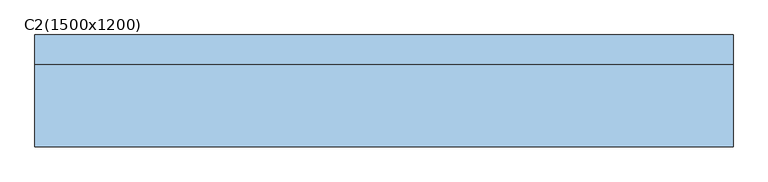
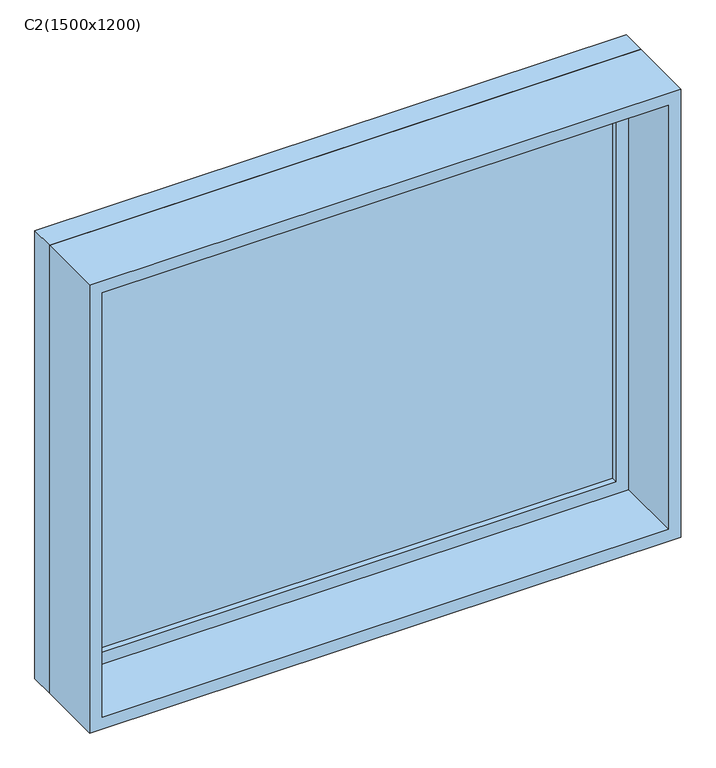
"""IFC4 building model written with IfcOpenShell, lengths in millimetres: window geometry, 固定窗 : C2(1500x1200)."""

import ifcopenshell
import ifcopenshell.guid

model = None  # the IFC model being written
_history = None  # IfcOwnerHistory: only IFC2X3 demands one
_inside = {}  # id of a spatial element -> (the spatial element, [elements in it])
_under = {}  # id of a project, library or spatial element -> (it, [spatial elements below it])
_declared = {}  # id of a project -> (the project, [libraries it declares])
_typed = {}  # id of a type object -> (the type object, [elements of that type])
_made_of = {}  # id of a material, layer set ... -> (it, [elements and type objects made of it])


def new_model(schema):
    """Start an empty IFC model of exactly this schema.

    Asked for "IFC4X3", IfcOpenShell would pick the latest addendum, in which some entities
    have other attributes; the version numbers below select the first issue.
    IFC2X3 requires an IfcOwnerHistory on every rooted entity: one is made here for all.
    """
    global model, _history
    if schema == "IFC4X3":
        model = ifcopenshell.file(schema_version=(4, 3, 0, 0))
    else:
        model = ifcopenshell.file(schema=schema)
    _inside.clear()
    _under.clear()
    _declared.clear()
    _typed.clear()
    _made_of.clear()
    _history = None
    if model.schema == "IFC2X3":
        org = make("IfcOrganization", Name="unknown")
        user = make(
            "IfcPersonAndOrganization",
            ThePerson=make("IfcPerson", FamilyName="unknown"),
            TheOrganization=org,
        )
        app = make(
            "IfcApplication",
            ApplicationDeveloper=org,
            Version="unknown",
            ApplicationFullName="unknown",
            ApplicationIdentifier="unknown",
        )
        _history = make(
            "IfcOwnerHistory",
            OwningUser=user,
            OwningApplication=app,
            ChangeAction="ADDED",
            CreationDate=0,
        )
    return model


def make(cls, **values):
    """One entity of the class cls with the attributes given. An attribute that is None is left unset."""
    return model.create_entity(
        cls, **{name: value for name, value in values.items() if value is not None}
    )


def rooted(cls, **values):
    """An entity with a GlobalId (a new one), such as an element, a storey or a relation."""
    return make(cls, GlobalId=ifcopenshell.guid.new(), OwnerHistory=_history, **values)


def si_unit(unit_type, name, prefix=None):
    """IfcSIUnit, for example si_unit("LENGTHUNIT", "METRE", prefix="MILLI")."""
    return make("IfcSIUnit", UnitType=unit_type, Prefix=prefix, Name=name)


def assignment(units):
    """IfcUnitAssignment: the units of a project."""
    return None if units is None else make("IfcUnitAssignment", Units=units)


def point(xyz):
    """IfcCartesianPoint."""
    return None if xyz is None else make("IfcCartesianPoint", Coordinates=xyz)


def direction(xyz):
    """IfcDirection."""
    return None if xyz is None else make("IfcDirection", DirectionRatios=xyz)


def frame(location, z_axis=None, x_axis=None):
    """IfcAxis2Placement3D, a coordinate frame: its origin and axes. An axis left out is left unset."""
    return make(
        "IfcAxis2Placement3D",
        Location=point(location),
        Axis=direction(z_axis),
        RefDirection=direction(x_axis),
    )


def origin():
    """The frame at (0, 0, 0) with its axes left unset."""
    return frame((0.0, 0.0, 0.0))


def place(relative_to, where):
    """IfcLocalPlacement: puts the frame where relative to a parent placement (None: the world)."""
    return make(
        "IfcLocalPlacement", PlacementRelTo=relative_to, RelativePlacement=where
    )


def context(
    kind, dimensions, precision=None, world=None, true_north=None, identifier=None
):
    """IfcGeometricRepresentationContext, for example the 3D "Model" context."""
    return make(
        "IfcGeometricRepresentationContext",
        ContextIdentifier=identifier,
        ContextType=kind,
        CoordinateSpaceDimension=dimensions,
        Precision=precision,
        WorldCoordinateSystem=world,
        TrueNorth=true_north,
    )


def project(units=None, contexts=None):
    """IfcProject with its units and contexts."""
    return rooted(
        "IfcProject",
        Name="project",
        RepresentationContexts=contexts,
        UnitsInContext=assignment(units),
    )


def spatial(cls, under=None, at=None, **own):
    """A site, building, storey or space (cls), placed at a placement, below another one or the project."""
    s = rooted(cls, ObjectPlacement=at, **own)
    if under is not None:
        _under.setdefault(under.id(), (under, []))[1].append(s)
    return s


def polyline(points):
    """IfcPolyline through the points."""
    return make("IfcPolyline", Points=[point(p) for p in points])


def outline(outer, holes=None, kind="AREA"):
    """IfcArbitraryClosedProfileDef: a profile drawn as a closed curve; with holes, ...WithVoids."""
    if holes is None:
        return make("IfcArbitraryClosedProfileDef", ProfileType=kind, OuterCurve=outer)
    return make(
        "IfcArbitraryProfileDefWithVoids",
        ProfileType=kind,
        OuterCurve=outer,
        InnerCurves=holes,
    )


def extrude(swept, where, along, depth):
    """IfcExtrudedAreaSolid: the profile swept, set in the frame where, extruded along a direction by depth."""
    return make(
        "IfcExtrudedAreaSolid",
        SweptArea=swept,
        Position=where,
        ExtrudedDirection=direction(along),
        Depth=depth,
    )


def shape(context_of_items, identifier, shape_type, items):
    """IfcShapeRepresentation: the items that make up one representation, for example the "Body"."""
    return make(
        "IfcShapeRepresentation",
        ContextOfItems=context_of_items,
        RepresentationIdentifier=identifier,
        RepresentationType=shape_type,
        Items=items,
    )


def source(mapping_origin, context_of_items, identifier, shape_type, items):
    """IfcRepresentationMap: a shape defined once, which mapped items show again and again."""
    return make(
        "IfcRepresentationMap",
        MappingOrigin=mapping_origin,
        MappedRepresentation=shape(context_of_items, identifier, shape_type, items),
    )


def transform(
    local_origin,
    x_axis=None,
    y_axis=None,
    z_axis=None,
    scale=None,
    scale2=None,
    scale3=None,
    uniform=True,
):
    """IfcCartesianTransformationOperator3D, or its non-uniform kind. x_axis, y_axis, z_axis: its Axis1, 2, 3."""
    if uniform:
        return make(
            "IfcCartesianTransformationOperator3D",
            Axis1=direction(x_axis),
            Axis2=direction(y_axis),
            LocalOrigin=point(local_origin),
            Scale=scale,
            Axis3=direction(z_axis),
        )
    return make(
        "IfcCartesianTransformationOperator3DnonUniform",
        Axis1=direction(x_axis),
        Axis2=direction(y_axis),
        LocalOrigin=point(local_origin),
        Scale=scale,
        Axis3=direction(z_axis),
        Scale2=scale2,
        Scale3=scale3,
    )


def mapped(mapping_source, mapping_target):
    """IfcMappedItem: shows the shape of a source again, moved by a transform."""
    return make(
        "IfcMappedItem", MappingSource=mapping_source, MappingTarget=mapping_target
    )


def made_of(thing, what):
    """Note that an element or type object is made of a material, layer set ...; save() writes the relation."""
    if what is not None:
        _made_of.setdefault(what.id(), (what, []))[1].append(thing)
    return thing


def element(
    cls,
    number,
    at=None,
    inside=None,
    cuts=None,
    type_object=None,
    material=None,
    context=None,
    identifier="Body",
    shape_type=None,
    held_by="IfcProductDefinitionShape",
    body=None,
    shapes=None,
    **own,
):
    """One element of the class cls, such as IfcWall. Its Tag is "e" and its number.

    at: its placement. inside: the storey or other place that contains it. cuts: it is an
    opening in that element (IfcRelVoidsElement). A single representation is given by context,
    identifier, shape_type and body (its items); several are given by shapes. held_by: the class
    of the entity that holds the representations. save() writes the other relations.
    """
    e = rooted(cls, Tag="e%d" % number, ObjectPlacement=at, **own)
    if body is not None:
        shapes = [shape(context, identifier, shape_type, body)]
    if shapes is not None:
        e.Representation = make(held_by, Representations=shapes)
    if inside is not None:
        _inside.setdefault(inside.id(), (inside, []))[1].append(e)
    if cuts is not None:
        rooted(
            "IfcRelVoidsElement", RelatingBuildingElement=cuts, RelatedOpeningElement=e
        )
    if type_object is not None:
        _typed.setdefault(type_object.id(), (type_object, []))[1].append(e)
    return made_of(e, material)


def aggregate(whole, parts):
    """IfcRelAggregates: a whole, such as a stair, and the parts it consists of."""
    return rooted("IfcRelAggregates", RelatingObject=whole, RelatedObjects=parts)


def save(model, path):
    """Write the relations noted so far, then the file.

    IfcRelAggregates (storeys below a building ...), IfcRelContainedInSpatialStructure (elements
    in a storey), IfcRelDefinesByType, IfcRelAssociatesMaterial and IfcRelDeclares: one each for
    every whole, place, type object, material and project.
    """
    for whole, parts in _under.values():
        aggregate(whole, parts)
    for where, things in _inside.values():
        rooted(
            "IfcRelContainedInSpatialStructure",
            RelatedElements=things,
            RelatingStructure=where,
        )
    for kind, things in _typed.values():
        rooted("IfcRelDefinesByType", RelatedObjects=things, RelatingType=kind)
    for what, things in _made_of.values():
        rooted("IfcRelAssociatesMaterial", RelatedObjects=things, RelatingMaterial=what)
    for by, libraries in _declared.values():
        rooted("IfcRelDeclares", RelatingContext=by, RelatedDefinitions=libraries)
    model.write(path)


def c2_1500x1200_cfff0f4c(model_context):
    return source(origin(), model_context, "Body", "SweptSolid", [
        extrude(outline(polyline([(648.4, 71.425), (-724.6, 71.425), (-724.6, 84.125), (648.4, 84.125), (648.4, 71.425)])), frame((0.0, 0.0, 963.5), z_axis=(0.0, 0.0, 1.0), x_axis=(1.0, 0.0, 0.0)), (0.0, 0.0, 1.0), 1073.0),
        extrude(outline(polyline([(2080.95, -769.05), (919.05, -769.05), (919.05, 692.85), (2080.95, 692.85), (2080.95, -769.05)]), holes=[polyline([(2036.5, -724.6), (2036.5, 648.4), (963.5, 648.4), (963.5, -724.6), (2036.5, -724.6)])]), frame((0.0, 55.55, 0.0), z_axis=(0.0, 1.0, 0.0), x_axis=(0.0, 0.0, 1.0)), (0.0, 0.0, 1.0), 44.45),
        extrude(outline(polyline([(2100.0, -788.1), (900.0, -788.1), (900.0, 711.9), (2100.0, 711.9), (2100.0, -788.1)]), holes=[polyline([(2068.25, -756.35), (2068.25, 680.15), (931.75, 680.15), (931.75, -756.35), (2068.25, -756.35)])]), frame((0.0, -120.0, 0.0), z_axis=(0.0, 1.0, 0.0), x_axis=(0.0, 0.0, 1.0)), (0.0, 0.0, 1.0), 175.55),
        extrude(outline(polyline([(2100.0, 711.9), (2100.0, -788.1), (900.0, -788.1), (900.0, 711.9), (2100.0, 711.9)]), holes=[polyline([(2080.95, 692.85), (919.05, 692.85), (919.05, -769.05), (2080.95, -769.05), (2080.95, 692.85)])]), frame((0.0, 55.55, 0.0), z_axis=(0.0, 1.0, 0.0), x_axis=(0.0, 0.0, 1.0)), (0.0, 0.0, 1.0), 64.45),
    ])


if __name__ == "__main__":
    model = new_model("IFC4")
    model_context = context("Model", 3, world=origin())
    ifc_project = project(units=[si_unit("LENGTHUNIT", "METRE", prefix="MILLI")], contexts=[model_context])
    site = spatial("IfcSite", under=ifc_project)
    building = spatial("IfcBuilding", under=site)
    placement = place(None, origin())
    c2_1500x1200_shape = c2_1500x1200_cfff0f4c(model_context)
    element("IfcWindow", 1, ObjectType="固定窗 : C2(1500x1200)", at=placement, inside=building, context=model_context, shape_type="MappedRepresentation", body=[
        mapped(c2_1500x1200_shape, transform((0.0, 0.0, 0.0), x_axis=(1.0, 0.0, 0.0), y_axis=(0.0, 1.0, 0.0), z_axis=(0.0, 0.0, 1.0))),
    ])
    save(model, "model.ifc")

# Revit data of these elements
# Type "固定窗 : C2(1500x1200)"
#   Type Mark = "C1517"
#   Construction Type Id = "SGL"
#   Analytic Construction = "大型单层玻璃窗"
#   Visual Light Transmittance = 0.9
#   Solar Heat Gain Coefficient = 0.86
#   Rough Width = 1500 mm
#   Rough Height = 1200 mm
#   Heat Transfer Coefficient (U) = 5.5617 W/(m²·K)
#   Height = 1200 mm
#   默认窗台高度 = 900 mm
#   Width = 1500 mm
#   窗嵌入 = 20 mm
#   高窗平面 [instance default] = no
#   通用窗平面 [instance default] = yes
#   玻璃 = none
#   框架材质 = none
#   Wall Closure = (empty or 0)
# Element 1 (IfcWindow, "固定窗 : C2(1500x1200)")
#   Materials on its faces: "玻璃"
# Materials
#   "玻璃": class "玻璃", colour RGB 0 128 192, transparency 0.9, Description = "钠钙玻璃", Cost = 0
